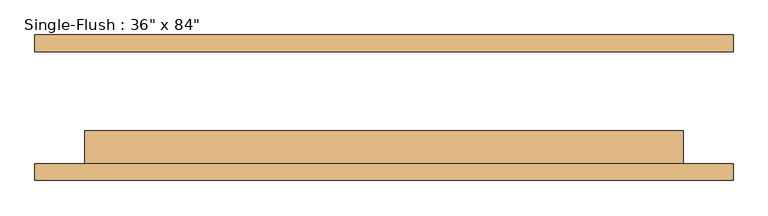
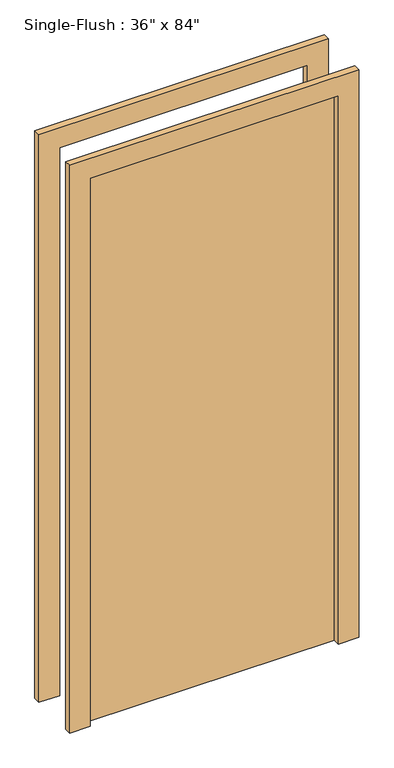
"""IFC4 building model written with IfcOpenShell, lengths in millimetres: door geometry."""

import ifcopenshell
import ifcopenshell.guid

model = None  # the IFC model being written
_history = None  # IfcOwnerHistory: only IFC2X3 demands one
_inside = {}  # id of a spatial element -> (the spatial element, [elements in it])
_under = {}  # id of a project, library or spatial element -> (it, [spatial elements below it])
_declared = {}  # id of a project -> (the project, [libraries it declares])
_typed = {}  # id of a type object -> (the type object, [elements of that type])
_made_of = {}  # id of a material, layer set ... -> (it, [elements and type objects made of it])


def new_model(schema):
    """Start an empty IFC model of exactly this schema.

    Asked for "IFC4X3", IfcOpenShell would pick the latest addendum, in which some entities
    have other attributes; the version numbers below select the first issue.
    IFC2X3 requires an IfcOwnerHistory on every rooted entity: one is made here for all.
    """
    global model, _history
    if schema == "IFC4X3":
        model = ifcopenshell.file(schema_version=(4, 3, 0, 0))
    else:
        model = ifcopenshell.file(schema=schema)
    _inside.clear()
    _under.clear()
    _declared.clear()
    _typed.clear()
    _made_of.clear()
    _history = None
    if model.schema == "IFC2X3":
        org = make("IfcOrganization", Name="unknown")
        user = make(
            "IfcPersonAndOrganization",
            ThePerson=make("IfcPerson", FamilyName="unknown"),
            TheOrganization=org,
        )
        app = make(
            "IfcApplication",
            ApplicationDeveloper=org,
            Version="unknown",
            ApplicationFullName="unknown",
            ApplicationIdentifier="unknown",
        )
        _history = make(
            "IfcOwnerHistory",
            OwningUser=user,
            OwningApplication=app,
            ChangeAction="ADDED",
            CreationDate=0,
        )
    return model


def make(cls, **values):
    """One entity of the class cls with the attributes given. An attribute that is None is left unset."""
    return model.create_entity(
        cls, **{name: value for name, value in values.items() if value is not None}
    )


def rooted(cls, **values):
    """An entity with a GlobalId (a new one), such as an element, a storey or a relation."""
    return make(cls, GlobalId=ifcopenshell.guid.new(), OwnerHistory=_history, **values)


def si_unit(unit_type, name, prefix=None):
    """IfcSIUnit, for example si_unit("LENGTHUNIT", "METRE", prefix="MILLI")."""
    return make("IfcSIUnit", UnitType=unit_type, Prefix=prefix, Name=name)


def assignment(units):
    """IfcUnitAssignment: the units of a project."""
    return None if units is None else make("IfcUnitAssignment", Units=units)


def point(xyz):
    """IfcCartesianPoint."""
    return None if xyz is None else make("IfcCartesianPoint", Coordinates=xyz)


def direction(xyz):
    """IfcDirection."""
    return None if xyz is None else make("IfcDirection", DirectionRatios=xyz)


def frame(location, z_axis=None, x_axis=None):
    """IfcAxis2Placement3D, a coordinate frame: its origin and axes. An axis left out is left unset."""
    return make(
        "IfcAxis2Placement3D",
        Location=point(location),
        Axis=direction(z_axis),
        RefDirection=direction(x_axis),
    )


def origin():
    """The frame at (0, 0, 0) with its axes left unset."""
    return frame((0.0, 0.0, 0.0))


def origin_with_axes():
    """The frame at (0, 0, 0) with the z axis (0, 0, 1) and the x axis (1, 0, 0) written out."""
    return frame((0.0, 0.0, 0.0), z_axis=(0.0, 0.0, 1.0), x_axis=(1.0, 0.0, 0.0))


def place(relative_to, where):
    """IfcLocalPlacement: puts the frame where relative to a parent placement (None: the world)."""
    return make(
        "IfcLocalPlacement", PlacementRelTo=relative_to, RelativePlacement=where
    )


def context(
    kind, dimensions, precision=None, world=None, true_north=None, identifier=None
):
    """IfcGeometricRepresentationContext, for example the 3D "Model" context."""
    return make(
        "IfcGeometricRepresentationContext",
        ContextIdentifier=identifier,
        ContextType=kind,
        CoordinateSpaceDimension=dimensions,
        Precision=precision,
        WorldCoordinateSystem=world,
        TrueNorth=true_north,
    )


def project(units=None, contexts=None):
    """IfcProject with its units and contexts."""
    return rooted(
        "IfcProject",
        Name="project",
        RepresentationContexts=contexts,
        UnitsInContext=assignment(units),
    )


def spatial(cls, under=None, at=None, **own):
    """A site, building, storey or space (cls), placed at a placement, below another one or the project."""
    s = rooted(cls, ObjectPlacement=at, **own)
    if under is not None:
        _under.setdefault(under.id(), (under, []))[1].append(s)
    return s


def polyline(points):
    """IfcPolyline through the points."""
    return make("IfcPolyline", Points=[point(p) for p in points])


def outline(outer, holes=None, kind="AREA"):
    """IfcArbitraryClosedProfileDef: a profile drawn as a closed curve; with holes, ...WithVoids."""
    if holes is None:
        return make("IfcArbitraryClosedProfileDef", ProfileType=kind, OuterCurve=outer)
    return make(
        "IfcArbitraryProfileDefWithVoids",
        ProfileType=kind,
        OuterCurve=outer,
        InnerCurves=holes,
    )


def extrude(swept, where, along, depth):
    """IfcExtrudedAreaSolid: the profile swept, set in the frame where, extruded along a direction by depth."""
    return make(
        "IfcExtrudedAreaSolid",
        SweptArea=swept,
        Position=where,
        ExtrudedDirection=direction(along),
        Depth=depth,
    )


def shape(context_of_items, identifier, shape_type, items):
    """IfcShapeRepresentation: the items that make up one representation, for example the "Body"."""
    return make(
        "IfcShapeRepresentation",
        ContextOfItems=context_of_items,
        RepresentationIdentifier=identifier,
        RepresentationType=shape_type,
        Items=items,
    )


def source(mapping_origin, context_of_items, identifier, shape_type, items):
    """IfcRepresentationMap: a shape defined once, which mapped items show again and again."""
    return make(
        "IfcRepresentationMap",
        MappingOrigin=mapping_origin,
        MappedRepresentation=shape(context_of_items, identifier, shape_type, items),
    )


def transform(
    local_origin,
    x_axis=None,
    y_axis=None,
    z_axis=None,
    scale=None,
    scale2=None,
    scale3=None,
    uniform=True,
):
    """IfcCartesianTransformationOperator3D, or its non-uniform kind. x_axis, y_axis, z_axis: its Axis1, 2, 3."""
    if uniform:
        return make(
            "IfcCartesianTransformationOperator3D",
            Axis1=direction(x_axis),
            Axis2=direction(y_axis),
            LocalOrigin=point(local_origin),
            Scale=scale,
            Axis3=direction(z_axis),
        )
    return make(
        "IfcCartesianTransformationOperator3DnonUniform",
        Axis1=direction(x_axis),
        Axis2=direction(y_axis),
        LocalOrigin=point(local_origin),
        Scale=scale,
        Axis3=direction(z_axis),
        Scale2=scale2,
        Scale3=scale3,
    )


def mapped(mapping_source, mapping_target):
    """IfcMappedItem: shows the shape of a source again, moved by a transform."""
    return make(
        "IfcMappedItem", MappingSource=mapping_source, MappingTarget=mapping_target
    )


def made_of(thing, what):
    """Note that an element or type object is made of a material, layer set ...; save() writes the relation."""
    if what is not None:
        _made_of.setdefault(what.id(), (what, []))[1].append(thing)
    return thing


def element(
    cls,
    number,
    at=None,
    inside=None,
    cuts=None,
    type_object=None,
    material=None,
    context=None,
    identifier="Body",
    shape_type=None,
    held_by="IfcProductDefinitionShape",
    body=None,
    shapes=None,
    **own,
):
    """One element of the class cls, such as IfcWall. Its Tag is "e" and its number.

    at: its placement. inside: the storey or other place that contains it. cuts: it is an
    opening in that element (IfcRelVoidsElement). A single representation is given by context,
    identifier, shape_type and body (its items); several are given by shapes. held_by: the class
    of the entity that holds the representations. save() writes the other relations.
    """
    e = rooted(cls, Tag="e%d" % number, ObjectPlacement=at, **own)
    if body is not None:
        shapes = [shape(context, identifier, shape_type, body)]
    if shapes is not None:
        e.Representation = make(held_by, Representations=shapes)
    if inside is not None:
        _inside.setdefault(inside.id(), (inside, []))[1].append(e)
    if cuts is not None:
        rooted(
            "IfcRelVoidsElement", RelatingBuildingElement=cuts, RelatedOpeningElement=e
        )
    if type_object is not None:
        _typed.setdefault(type_object.id(), (type_object, []))[1].append(e)
    return made_of(e, material)


def aggregate(whole, parts):
    """IfcRelAggregates: a whole, such as a stair, and the parts it consists of."""
    return rooted("IfcRelAggregates", RelatingObject=whole, RelatedObjects=parts)


def save(model, path):
    """Write the relations noted so far, then the file.

    IfcRelAggregates (storeys below a building ...), IfcRelContainedInSpatialStructure (elements
    in a storey), IfcRelDefinesByType, IfcRelAssociatesMaterial and IfcRelDeclares: one each for
    every whole, place, type object, material and project.
    """
    for whole, parts in _under.values():
        aggregate(whole, parts)
    for where, things in _inside.values():
        rooted(
            "IfcRelContainedInSpatialStructure",
            RelatedElements=things,
            RelatingStructure=where,
        )
    for kind, things in _typed.values():
        rooted("IfcRelDefinesByType", RelatedObjects=things, RelatingType=kind)
    for what, things in _made_of.values():
        rooted("IfcRelAssociatesMaterial", RelatedObjects=things, RelatingMaterial=what)
    for by, libraries in _declared.values():
        rooted("IfcRelDeclares", RelatingContext=by, RelatedDefinitions=libraries)
    model.write(path)


def door_d7907053(model_context):
    return source(origin(), model_context, "Body", "SweptSolid", [
        extrude(outline(polyline([(2209.8, -533.4), (0.0, -533.4), (0.0, -457.2), (2133.6, -457.2), (2133.6, 457.2), (0.0, 457.2), (0.0, 533.4), (2209.8, 533.4), (2209.8, -533.4)])), frame((0.0, -111.125, 0.0), z_axis=(0.0, 1.0, 0.0), x_axis=(0.0, 0.0, 1.0)), (0.0, 0.0, 1.0), 25.4),
        extrude(outline(polyline([(2209.8, 533.4), (2209.8, -533.4), (0.0, -533.4), (0.0, -457.2), (2133.6, -457.2), (2133.6, 457.2), (0.0, 457.2), (0.0, 533.4), (2209.8, 533.4)])), frame((0.0, 85.725, 0.0), z_axis=(0.0, 1.0, 0.0), x_axis=(0.0, 0.0, 1.0)), (0.0, 0.0, 1.0), 25.4),
        extrude(outline(polyline([(457.2, -34.925), (457.2, -85.725), (-457.2, -85.725), (-457.2, -34.925), (457.2, -34.925)])), origin_with_axes(), (0.0, 0.0, 1.0), 2133.6),
    ])


if __name__ == "__main__":
    model = new_model("IFC4")
    model_context = context("Model", 3, world=origin())
    ifc_project = project(units=[si_unit("LENGTHUNIT", "METRE", prefix="MILLI")], contexts=[model_context])
    site = spatial("IfcSite", under=ifc_project)
    building = spatial("IfcBuilding", under=site)
    placement = place(None, origin())
    door_shape = door_d7907053(model_context)
    element("IfcDoor", 1, ObjectType="Single-Flush : 36\" x 84\"", at=placement, inside=building, context=model_context, shape_type="MappedRepresentation", body=[
        mapped(door_shape, transform((0.0, 0.0, 0.0), x_axis=(1.0, 0.0, 0.0), y_axis=(0.0, 1.0, 0.0), z_axis=(0.0, 0.0, 1.0))),
    ])
    save(model, "model.ifc")

# Revit data of these elements
# Type "Single-Flush : 36\" x 84\""
#   Type Mark = "1"
#   Assembly Code = "C1020"
#   Thickness = 0' - 2"
#   Height = 7' - 0"
#   Trim Projection Ext = 0' - 1"
#   Trim Projection Int = 0' - 1"
#   Trim Width = 0' - 3"
#   Width = 3' - 0"
#   Door Material = none
#   Frame Material = none
#   Function = (empty or 0)
#   Wall Closure = (empty or 0)
